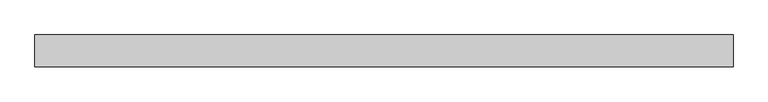
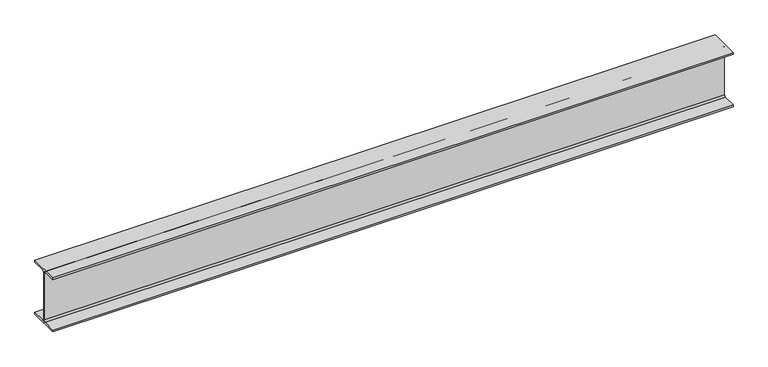
"""IFC4 building model written with IfcOpenShell, lengths in millimetres: beam geometry, Old_Steel Beam_H-KSD3502 : H_SB_ASB_H-250×125x6x9."""

from ifc_helpers import new_model, si_unit, point, frame, frame_2d, origin, place, context, project, spatial, polyline, circle_curve, trimmed, segment, composite_curve, outline, extrude, source, transform, mapped, element, save


def beam_bc66176e(model_context):
    return source(origin(), model_context, "Body", "SweptSolid", [
        extrude(outline(composite_curve([segment(polyline([(82.5, -141.5), (82.5, -151.7), (-82.5, -151.7), (-82.5, -141.5), (-11.9, -141.5)]), True, "CONTINUOUS"), segment(trimmed(circle_curve(frame_2d((-11.9, -132.6)), 8.9), [point((-11.9, -141.5))], [point((-3.0, -132.6))], True, "CARTESIAN"), True, "CONTINUOUS"), segment(polyline([(-3.0, -132.6), (-3.0, 132.6)]), True, "CONTINUOUS"), segment(trimmed(circle_curve(frame_2d((-11.9, 132.6)), 8.9), [point((-3.0, 132.6))], [point((-11.9, 141.5))], True, "CARTESIAN"), True, "CONTINUOUS"), segment(polyline([(-11.9, 141.5), (-82.5, 141.5), (-82.5, 151.7), (82.5, 151.7), (82.5, 141.5), (11.9, 141.5)]), True, "CONTINUOUS"), segment(trimmed(circle_curve(frame_2d((11.9, 132.6)), 8.9), [point((11.9, 141.5))], [point((3.0, 132.6))], True, "CARTESIAN"), True, "CONTINUOUS"), segment(polyline([(3.0, 132.6), (3.0, -132.6)]), True, "CONTINUOUS"), segment(trimmed(circle_curve(frame_2d((11.9, -132.6)), 8.9), [point((3.0, -132.6))], [point((11.9, -141.5))], True, "CARTESIAN"), True, "CONTINUOUS"), segment(polyline([(11.9, -141.5), (82.5, -141.5)]), True, "CONTINUOUS")], self_intersect=False)), frame((-1904.8, 0.0, 0.0), z_axis=(1.0, 0.0, 0.0), x_axis=(0.0, 1.0, 0.0)), (0.0, 0.0, 1.0), 3623.1833333),
    ])


if __name__ == "__main__":
    model = new_model("IFC4")
    model_context = context("Model", 3, world=origin())
    ifc_project = project(units=[si_unit("LENGTHUNIT", "METRE", prefix="MILLI")], contexts=[model_context])
    site = spatial("IfcSite", under=ifc_project)
    building = spatial("IfcBuilding", under=site)
    placement = place(None, origin())
    beam_shape = beam_bc66176e(model_context)
    element("IfcBeam", 1, ObjectType="Old_Steel Beam_H-KSD3502 : H_SB_ASB_H-250×125x6x9", at=placement, inside=building, context=model_context, shape_type="MappedRepresentation", body=[
        mapped(beam_shape, transform((0.0, 0.0, 0.0), x_axis=(1.0, 0.0, 0.0), y_axis=(0.0, 1.0, 0.0), z_axis=(0.0, 0.0, 1.0))),
    ])
    save(model, "model.ifc")

# Revit data of these elements
# Type "Old_Steel Beam_H-KSD3502 : H_SB_ASB_H-250×125x6x9"
#   Width = 12.5 cm
#   Web Thickness = 0.6 cm
#   Web Fillet = 1.2 cm
#   Warping Constant = 42539.8 cm⁶
#   Torsional Moment of Inertia = 7.8102 cm⁴
#   Torsional Modulus = 1.0 cm³
#   Section Area = 37.66 cm²
#   Plastic Modulus weak axis = 73.1 cm³
#   Plastic Modulus strong axis = 366.0 cm³
#   Perimeter = 0.97 m²/m
#   Nominal Weight = 29.60 kgf/m
#   Moment of Inertia weak axis = 294.00 cm⁴
#   Moment of Inertia strong axis = 4050.00 cm⁴
#   Height = 25.0 cm
#   Flange Thickness = 0.9 cm
#   Elastic Modulus weak axis = 47.0 cm³
#   Elastic Modulus strong axis = 324.0 cm³
#   Centroid Vertical = 12.5 cm
#   Centroid Horizontal = 6.25 cm
#   Length [instance default] = 1.5240 m
#   Structural Material [instance default] = Steel, 45-345
#   Assembly Code = ""
# Element 1 (IfcBeam, "Old_Steel Beam_H-KSD3502 : H_SB_ASB_H-250×125x6x9")
#   Structural Material = none
# Materials
#   "Steel, 45-345": class "Metal", colour RGB 189 187 185, transparency 0, Description = "Steel 345 MPa", Cost = 0
